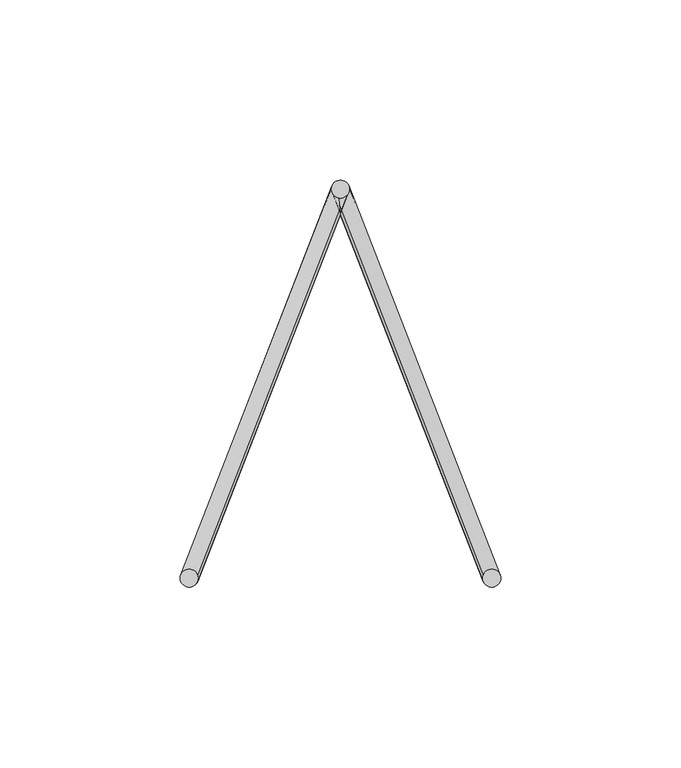
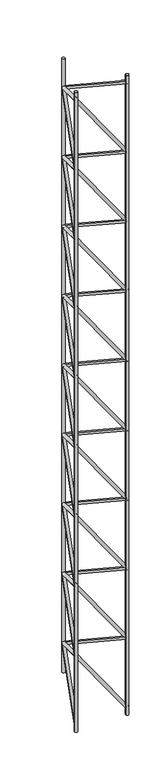
"""IFC4 building model written with IfcOpenShell, lengths in millimetres: proxy geometry, Pre-fab. (Vigota 3 - Pano 8)."""

from ifc_helpers import new_model, si_unit, point, frame, frame_2d, origin, origin_with_axes, origin_2d, place, context, project, spatial, circle_curve, trimmed, segment, composite_curve, outline, extrude, source, transform, mapped, element, save


def structural_framing_089a5535(model_context):
    return source(origin(), model_context, "Body", "SweptSolid", [
        extrude(outline(composite_curve([segment(trimmed(circle_curve(origin_2d(), 2.5), [point((2.5, 0.0))], [point((-2.5, 0.0))], False, "CARTESIAN"), True, "CONTINUOUS"), segment(trimmed(circle_curve(origin_2d(), 2.5), [point((-2.5, 0.0))], [point((2.5, 0.0))], False, "CARTESIAN"), True, "CONTINUOUS")], self_intersect=False)), origin_with_axes(), (0.0, 0.0, 1.0), 1105.691264),
        extrude(outline(composite_curve([segment(trimmed(circle_curve(frame_2d((-42.0, 108.0)), 2.5), [point((-39.5, 108.0))], [point((-44.5, 108.0))], False, "CARTESIAN"), True, "CONTINUOUS"), segment(trimmed(circle_curve(frame_2d((-42.0, 108.0)), 2.5), [point((-44.5, 108.0))], [point((-39.5, 108.0))], False, "CARTESIAN"), True, "CONTINUOUS")], self_intersect=False)), frame((0.0, 0.0, 22.8456318), z_axis=(0.0, 0.0, 1.0), x_axis=(1.0, 0.0, 0.0)), (0.0, 0.0, 1.0), 1060.0),
        extrude(outline(composite_curve([segment(trimmed(circle_curve(origin_2d(), 2.5), [point((2.5, 0.0))], [point((-2.5, 0.0))], False, "CARTESIAN"), True, "CONTINUOUS"), segment(trimmed(circle_curve(origin_2d(), 2.5), [point((-2.5, 0.0))], [point((2.5, 0.0))], False, "CARTESIAN"), True, "CONTINUOUS")], self_intersect=False)), frame((0.0, 0.0, 12.8456318), z_axis=(-0.3218603428886276, 0.8276408817707567, 0.4598004898837537), x_axis=(0.8192319205108605, -3.936835275445103e-11, 0.5734623443750141)), (0.0, 0.0, 1.0), 130.491379),
        extrude(outline(composite_curve([segment(trimmed(circle_curve(origin_2d(), 2.5), [point((2.5, 0.0))], [point((-2.5, 0.0))], False, "CARTESIAN"), True, "CONTINUOUS"), segment(trimmed(circle_curve(origin_2d(), 2.5), [point((-2.5, 0.0))], [point((2.5, 0.0))], False, "CARTESIAN"), True, "CONTINUOUS")], self_intersect=False)), frame((-42.0, 108.0, 72.8456318), z_axis=(0.3218603428886276, -0.8276408817707567, 0.4598004898837537), x_axis=(0.8192319205108605, -3.936835275445103e-11, -0.5734623443750141)), (0.0, 0.0, 1.0), 130.491379),
        extrude(outline(composite_curve([segment(trimmed(circle_curve(origin_2d(), 2.5), [point((2.5, 0.0))], [point((-2.5, 0.0))], False, "CARTESIAN"), True, "CONTINUOUS"), segment(trimmed(circle_curve(origin_2d(), 2.5), [point((-2.5, 0.0))], [point((2.5, 0.0))], False, "CARTESIAN"), True, "CONTINUOUS")], self_intersect=False)), frame((0.0, 0.0, 132.8456318), z_axis=(-0.3218603428886276, 0.8276408817707567, 0.4598004898837537), x_axis=(0.8192319205108605, -3.936835275445103e-11, 0.5734623443750141)), (0.0, 0.0, 1.0), 130.491379),
        extrude(outline(composite_curve([segment(trimmed(circle_curve(origin_2d(), 2.5), [point((2.5, 0.0))], [point((-2.5, 0.0))], False, "CARTESIAN"), True, "CONTINUOUS"), segment(trimmed(circle_curve(origin_2d(), 2.5), [point((-2.5, 0.0))], [point((2.5, 0.0))], False, "CARTESIAN"), True, "CONTINUOUS")], self_intersect=False)), frame((-42.0, 108.0, 192.8456318), z_axis=(0.3218603428886276, -0.8276408817707567, 0.4598004898837537), x_axis=(0.8192319205108605, -3.936835275445103e-11, -0.5734623443750141)), (0.0, 0.0, 1.0), 130.491379),
        extrude(outline(composite_curve([segment(trimmed(circle_curve(origin_2d(), 2.5), [point((2.5, 0.0))], [point((-2.5, 0.0))], False, "CARTESIAN"), True, "CONTINUOUS"), segment(trimmed(circle_curve(origin_2d(), 2.5), [point((-2.5, 0.0))], [point((2.5, 0.0))], False, "CARTESIAN"), True, "CONTINUOUS")], self_intersect=False)), frame((0.0, 0.0, 252.8456318), z_axis=(-0.3218603428886276, 0.8276408817707567, 0.4598004898837537), x_axis=(0.8192319205108605, -3.936835275445103e-11, 0.5734623443750141)), (0.0, 0.0, 1.0), 130.491379),
        extrude(outline(composite_curve([segment(trimmed(circle_curve(origin_2d(), 2.5), [point((2.5, 0.0))], [point((-2.5, 0.0))], False, "CARTESIAN"), True, "CONTINUOUS"), segment(trimmed(circle_curve(origin_2d(), 2.5), [point((-2.5, 0.0))], [point((2.5, 0.0))], False, "CARTESIAN"), True, "CONTINUOUS")], self_intersect=False)), frame((-42.0, 108.0, 312.8456318), z_axis=(0.3218603428886276, -0.8276408817707567, 0.4598004898837537), x_axis=(0.8192319205108605, -3.936835275445103e-11, -0.5734623443750141)), (0.0, 0.0, 1.0), 130.491379),
        extrude(outline(composite_curve([segment(trimmed(circle_curve(origin_2d(), 2.5), [point((2.5, 0.0))], [point((-2.5, 0.0))], False, "CARTESIAN"), True, "CONTINUOUS"), segment(trimmed(circle_curve(origin_2d(), 2.5), [point((-2.5, 0.0))], [point((2.5, 0.0))], False, "CARTESIAN"), True, "CONTINUOUS")], self_intersect=False)), frame((0.0, 0.0, 372.8456318), z_axis=(-0.3218603428886276, 0.8276408817707567, 0.4598004898837537), x_axis=(0.8192319205108605, -3.936835275445103e-11, 0.5734623443750141)), (0.0, 0.0, 1.0), 130.491379),
        extrude(outline(composite_curve([segment(trimmed(circle_curve(origin_2d(), 2.5), [point((2.5, 0.0))], [point((-2.5, 0.0))], False, "CARTESIAN"), True, "CONTINUOUS"), segment(trimmed(circle_curve(origin_2d(), 2.5), [point((-2.5, 0.0))], [point((2.5, 0.0))], False, "CARTESIAN"), True, "CONTINUOUS")], self_intersect=False)), frame((-42.0, 108.0, 432.8456318), z_axis=(0.3218603428886276, -0.8276408817707567, 0.4598004898837537), x_axis=(0.8192319205108605, -3.936835275445103e-11, -0.5734623443750141)), (0.0, 0.0, 1.0), 130.491379),
        extrude(outline(composite_curve([segment(trimmed(circle_curve(origin_2d(), 2.5), [point((2.5, 0.0))], [point((-2.5, 0.0))], False, "CARTESIAN"), True, "CONTINUOUS"), segment(trimmed(circle_curve(origin_2d(), 2.5), [point((-2.5, 0.0))], [point((2.5, 0.0))], False, "CARTESIAN"), True, "CONTINUOUS")], self_intersect=False)), frame((0.0, 0.0, 492.8456318), z_axis=(-0.3218603428886276, 0.8276408817707567, 0.4598004898837537), x_axis=(0.8192319205108605, -3.936835275445103e-11, 0.5734623443750141)), (0.0, 0.0, 1.0), 130.491379),
        extrude(outline(composite_curve([segment(trimmed(circle_curve(origin_2d(), 2.5), [point((2.5, 0.0))], [point((-2.5, 0.0))], False, "CARTESIAN"), True, "CONTINUOUS"), segment(trimmed(circle_curve(origin_2d(), 2.5), [point((-2.5, 0.0))], [point((2.5, 0.0))], False, "CARTESIAN"), True, "CONTINUOUS")], self_intersect=False)), frame((-42.0, 108.0, 552.8456318), z_axis=(0.3218603428886276, -0.8276408817707567, 0.4598004898837537), x_axis=(0.8192319205108605, -3.936835275445103e-11, -0.5734623443750141)), (0.0, 0.0, 1.0), 130.491379),
        extrude(outline(composite_curve([segment(trimmed(circle_curve(origin_2d(), 2.5), [point((2.5, 0.0))], [point((-2.5, 0.0))], False, "CARTESIAN"), True, "CONTINUOUS"), segment(trimmed(circle_curve(origin_2d(), 2.5), [point((-2.5, 0.0))], [point((2.5, 0.0))], False, "CARTESIAN"), True, "CONTINUOUS")], self_intersect=False)), frame((0.0, 0.0, 612.8456318), z_axis=(-0.3218603428886276, 0.8276408817707567, 0.4598004898837537), x_axis=(0.8192319205108605, -3.936835275445103e-11, 0.5734623443750141)), (0.0, 0.0, 1.0), 130.491379),
        extrude(outline(composite_curve([segment(trimmed(circle_curve(origin_2d(), 2.5), [point((2.5, 0.0))], [point((-2.5, 0.0))], False, "CARTESIAN"), True, "CONTINUOUS"), segment(trimmed(circle_curve(origin_2d(), 2.5), [point((-2.5, 0.0))], [point((2.5, 0.0))], False, "CARTESIAN"), True, "CONTINUOUS")], self_intersect=False)), frame((-42.0, 108.0, 672.8456318), z_axis=(0.3218603428886276, -0.8276408817707567, 0.4598004898837537), x_axis=(0.8192319205108605, -3.936835275445103e-11, -0.5734623443750141)), (0.0, 0.0, 1.0), 130.491379),
        extrude(outline(composite_curve([segment(trimmed(circle_curve(origin_2d(), 2.5), [point((2.5, 0.0))], [point((-2.5, 0.0))], False, "CARTESIAN"), True, "CONTINUOUS"), segment(trimmed(circle_curve(origin_2d(), 2.5), [point((-2.5, 0.0))], [point((2.5, 0.0))], False, "CARTESIAN"), True, "CONTINUOUS")], self_intersect=False)), frame((0.0, 0.0, 732.8456318), z_axis=(-0.3218603428886276, 0.8276408817707567, 0.4598004898837537), x_axis=(0.8192319205108605, -3.936835275445103e-11, 0.5734623443750141)), (0.0, 0.0, 1.0), 130.491379),
        extrude(outline(composite_curve([segment(trimmed(circle_curve(origin_2d(), 2.5), [point((2.5, 0.0))], [point((-2.5, 0.0))], False, "CARTESIAN"), True, "CONTINUOUS"), segment(trimmed(circle_curve(origin_2d(), 2.5), [point((-2.5, 0.0))], [point((2.5, 0.0))], False, "CARTESIAN"), True, "CONTINUOUS")], self_intersect=False)), frame((-42.0, 108.0, 792.8456318), z_axis=(0.3218603428886276, -0.8276408817707567, 0.4598004898837537), x_axis=(0.8192319205108605, -3.936835275445103e-11, -0.5734623443750141)), (0.0, 0.0, 1.0), 130.491379),
        extrude(outline(composite_curve([segment(trimmed(circle_curve(origin_2d(), 2.5), [point((2.5, 0.0))], [point((-2.5, 0.0))], False, "CARTESIAN"), True, "CONTINUOUS"), segment(trimmed(circle_curve(origin_2d(), 2.5), [point((-2.5, 0.0))], [point((2.5, 0.0))], False, "CARTESIAN"), True, "CONTINUOUS")], self_intersect=False)), frame((0.0, 0.0, 852.8456318), z_axis=(-0.3218603428886276, 0.8276408817707567, 0.4598004898837537), x_axis=(0.8192319205108605, -3.936835275445103e-11, 0.5734623443750141)), (0.0, 0.0, 1.0), 130.491379),
        extrude(outline(composite_curve([segment(trimmed(circle_curve(origin_2d(), 2.5), [point((2.5, 0.0))], [point((-2.5, 0.0))], False, "CARTESIAN"), True, "CONTINUOUS"), segment(trimmed(circle_curve(origin_2d(), 2.5), [point((-2.5, 0.0))], [point((2.5, 0.0))], False, "CARTESIAN"), True, "CONTINUOUS")], self_intersect=False)), frame((-42.0, 108.0, 912.8456318), z_axis=(0.3218603428886276, -0.8276408817707567, 0.4598004898837537), x_axis=(0.8192319205108605, -3.936835275445103e-11, -0.5734623443750141)), (0.0, 0.0, 1.0), 130.491379),
        extrude(outline(composite_curve([segment(trimmed(circle_curve(origin_2d(), 2.5), [point((2.5, 0.0))], [point((-2.5, 0.0))], False, "CARTESIAN"), True, "CONTINUOUS"), segment(trimmed(circle_curve(origin_2d(), 2.5), [point((-2.5, 0.0))], [point((2.5, 0.0))], False, "CARTESIAN"), True, "CONTINUOUS")], self_intersect=False)), frame((0.0, 0.0, 972.8456318), z_axis=(-0.3218603428886276, 0.8276408817707567, 0.4598004898837537), x_axis=(0.8192319205108605, -3.936835275445103e-11, 0.5734623443750141)), (0.0, 0.0, 1.0), 130.491379),
        extrude(outline(composite_curve([segment(trimmed(circle_curve(origin_2d(), 2.5), [point((2.5, 0.0))], [point((-2.5, 0.0))], False, "CARTESIAN"), True, "CONTINUOUS"), segment(trimmed(circle_curve(origin_2d(), 2.5), [point((-2.5, 0.0))], [point((2.5, 0.0))], False, "CARTESIAN"), True, "CONTINUOUS")], self_intersect=False)), frame((-42.0, 108.0, 1032.845632), z_axis=(0.3218603428886276, -0.8276408817707567, 0.4598004898837537), x_axis=(0.8192319205108605, -3.936835275445103e-11, -0.5734623443750141)), (0.0, 0.0, 1.0), 130.491379),
        extrude(outline(composite_curve([segment(trimmed(circle_curve(frame_2d((-84.0, 0.0)), 2.5), [point((-81.5, 0.0))], [point((-86.5, 0.0))], False, "CARTESIAN"), True, "CONTINUOUS"), segment(trimmed(circle_curve(frame_2d((-84.0, 0.0)), 2.5), [point((-86.5, 0.0))], [point((-81.5, 0.0))], False, "CARTESIAN"), True, "CONTINUOUS")], self_intersect=False)), origin_with_axes(), (0.0, 0.0, 1.0), 1105.691264),
        extrude(outline(composite_curve([segment(trimmed(circle_curve(origin_2d(), 2.5), [point((2.5, 0.0))], [point((-2.5, 0.0))], False, "CARTESIAN"), True, "CONTINUOUS"), segment(trimmed(circle_curve(origin_2d(), 2.5), [point((-2.5, 0.0))], [point((2.5, 0.0))], False, "CARTESIAN"), True, "CONTINUOUS")], self_intersect=False)), frame((-84.0, 0.0, 12.8456318), z_axis=(0.3218603428886276, 0.8276408817707567, 0.4598004898837537), x_axis=(0.8192319205108605, 3.936835275445103e-11, -0.5734623443750141)), (0.0, 0.0, 1.0), 130.491379),
        extrude(outline(composite_curve([segment(trimmed(circle_curve(origin_2d(), 2.5), [point((2.5, 0.0))], [point((-2.5, 0.0))], False, "CARTESIAN"), True, "CONTINUOUS"), segment(trimmed(circle_curve(origin_2d(), 2.5), [point((-2.5, 0.0))], [point((2.5, 0.0))], False, "CARTESIAN"), True, "CONTINUOUS")], self_intersect=False)), frame((-42.0, 108.0, 72.8456318), z_axis=(-0.3218603428886276, -0.8276408817707567, 0.4598004898837537), x_axis=(0.8192319205108605, 3.936835275445103e-11, 0.5734623443750141)), (0.0, 0.0, 1.0), 130.491379),
        extrude(outline(composite_curve([segment(trimmed(circle_curve(origin_2d(), 2.5), [point((2.5, 0.0))], [point((-2.5, 0.0))], False, "CARTESIAN"), True, "CONTINUOUS"), segment(trimmed(circle_curve(origin_2d(), 2.5), [point((-2.5, 0.0))], [point((2.5, 0.0))], False, "CARTESIAN"), True, "CONTINUOUS")], self_intersect=False)), frame((-84.0, 0.0, 132.8456318), z_axis=(0.3218603428886276, 0.8276408817707567, 0.4598004898837537), x_axis=(0.8192319205108605, 3.936835275445103e-11, -0.5734623443750141)), (0.0, 0.0, 1.0), 130.491379),
        extrude(outline(composite_curve([segment(trimmed(circle_curve(origin_2d(), 2.5), [point((2.5, 0.0))], [point((-2.5, 0.0))], False, "CARTESIAN"), True, "CONTINUOUS"), segment(trimmed(circle_curve(origin_2d(), 2.5), [point((-2.5, 0.0))], [point((2.5, 0.0))], False, "CARTESIAN"), True, "CONTINUOUS")], self_intersect=False)), frame((-42.0, 108.0, 192.8456318), z_axis=(-0.3218603428886276, -0.8276408817707567, 0.4598004898837537), x_axis=(0.8192319205108605, 3.936835275445103e-11, 0.5734623443750141)), (0.0, 0.0, 1.0), 130.491379),
        extrude(outline(composite_curve([segment(trimmed(circle_curve(origin_2d(), 2.5), [point((2.5, 0.0))], [point((-2.5, 0.0))], False, "CARTESIAN"), True, "CONTINUOUS"), segment(trimmed(circle_curve(origin_2d(), 2.5), [point((-2.5, 0.0))], [point((2.5, 0.0))], False, "CARTESIAN"), True, "CONTINUOUS")], self_intersect=False)), frame((-84.0, 0.0, 252.8456318), z_axis=(0.3218603428886276, 0.8276408817707567, 0.4598004898837537), x_axis=(0.8192319205108605, 3.936835275445103e-11, -0.5734623443750141)), (0.0, 0.0, 1.0), 130.491379),
        extrude(outline(composite_curve([segment(trimmed(circle_curve(origin_2d(), 2.5), [point((2.5, 0.0))], [point((-2.5, 0.0))], False, "CARTESIAN"), True, "CONTINUOUS"), segment(trimmed(circle_curve(origin_2d(), 2.5), [point((-2.5, 0.0))], [point((2.5, 0.0))], False, "CARTESIAN"), True, "CONTINUOUS")], self_intersect=False)), frame((-42.0, 108.0, 312.8456318), z_axis=(-0.3218603428886276, -0.8276408817707567, 0.4598004898837537), x_axis=(0.8192319205108605, 3.936835275445103e-11, 0.5734623443750141)), (0.0, 0.0, 1.0), 130.491379),
        extrude(outline(composite_curve([segment(trimmed(circle_curve(origin_2d(), 2.5), [point((2.5, 0.0))], [point((-2.5, 0.0))], False, "CARTESIAN"), True, "CONTINUOUS"), segment(trimmed(circle_curve(origin_2d(), 2.5), [point((-2.5, 0.0))], [point((2.5, 0.0))], False, "CARTESIAN"), True, "CONTINUOUS")], self_intersect=False)), frame((-84.0, 0.0, 372.8456318), z_axis=(0.3218603428886276, 0.8276408817707567, 0.4598004898837537), x_axis=(0.8192319205108605, 3.936835275445103e-11, -0.5734623443750141)), (0.0, 0.0, 1.0), 130.491379),
        extrude(outline(composite_curve([segment(trimmed(circle_curve(origin_2d(), 2.5), [point((2.5, 0.0))], [point((-2.5, 0.0))], False, "CARTESIAN"), True, "CONTINUOUS"), segment(trimmed(circle_curve(origin_2d(), 2.5), [point((-2.5, 0.0))], [point((2.5, 0.0))], False, "CARTESIAN"), True, "CONTINUOUS")], self_intersect=False)), frame((-42.0, 108.0, 432.8456318), z_axis=(-0.3218603428886276, -0.8276408817707567, 0.4598004898837537), x_axis=(0.8192319205108605, 3.936835275445103e-11, 0.5734623443750141)), (0.0, 0.0, 1.0), 130.491379),
        extrude(outline(composite_curve([segment(trimmed(circle_curve(origin_2d(), 2.5), [point((2.5, 0.0))], [point((-2.5, 0.0))], False, "CARTESIAN"), True, "CONTINUOUS"), segment(trimmed(circle_curve(origin_2d(), 2.5), [point((-2.5, 0.0))], [point((2.5, 0.0))], False, "CARTESIAN"), True, "CONTINUOUS")], self_intersect=False)), frame((-84.0, 0.0, 492.8456318), z_axis=(0.3218603428886276, 0.8276408817707567, 0.4598004898837537), x_axis=(0.8192319205108605, 3.936835275445103e-11, -0.5734623443750141)), (0.0, 0.0, 1.0), 130.491379),
        extrude(outline(composite_curve([segment(trimmed(circle_curve(origin_2d(), 2.5), [point((2.5, 0.0))], [point((-2.5, 0.0))], False, "CARTESIAN"), True, "CONTINUOUS"), segment(trimmed(circle_curve(origin_2d(), 2.5), [point((-2.5, 0.0))], [point((2.5, 0.0))], False, "CARTESIAN"), True, "CONTINUOUS")], self_intersect=False)), frame((-42.0, 108.0, 552.8456318), z_axis=(-0.3218603428886276, -0.8276408817707567, 0.4598004898837537), x_axis=(0.8192319205108605, 3.936835275445103e-11, 0.5734623443750141)), (0.0, 0.0, 1.0), 130.491379),
        extrude(outline(composite_curve([segment(trimmed(circle_curve(origin_2d(), 2.5), [point((2.5, 0.0))], [point((-2.5, 0.0))], False, "CARTESIAN"), True, "CONTINUOUS"), segment(trimmed(circle_curve(origin_2d(), 2.5), [point((-2.5, 0.0))], [point((2.5, 0.0))], False, "CARTESIAN"), True, "CONTINUOUS")], self_intersect=False)), frame((-84.0, 0.0, 612.8456318), z_axis=(0.3218603428886276, 0.8276408817707567, 0.4598004898837537), x_axis=(0.8192319205108605, 3.936835275445103e-11, -0.5734623443750141)), (0.0, 0.0, 1.0), 130.491379),
        extrude(outline(composite_curve([segment(trimmed(circle_curve(origin_2d(), 2.5), [point((2.5, 0.0))], [point((-2.5, 0.0))], False, "CARTESIAN"), True, "CONTINUOUS"), segment(trimmed(circle_curve(origin_2d(), 2.5), [point((-2.5, 0.0))], [point((2.5, 0.0))], False, "CARTESIAN"), True, "CONTINUOUS")], self_intersect=False)), frame((-42.0, 108.0, 672.8456318), z_axis=(-0.3218603428886276, -0.8276408817707567, 0.4598004898837537), x_axis=(0.8192319205108605, 3.936835275445103e-11, 0.5734623443750141)), (0.0, 0.0, 1.0), 130.491379),
        extrude(outline(composite_curve([segment(trimmed(circle_curve(origin_2d(), 2.5), [point((2.5, 0.0))], [point((-2.5, 0.0))], False, "CARTESIAN"), True, "CONTINUOUS"), segment(trimmed(circle_curve(origin_2d(), 2.5), [point((-2.5, 0.0))], [point((2.5, 0.0))], False, "CARTESIAN"), True, "CONTINUOUS")], self_intersect=False)), frame((-84.0, 0.0, 732.8456318), z_axis=(0.3218603428886276, 0.8276408817707567, 0.4598004898837537), x_axis=(0.8192319205108605, 3.936835275445103e-11, -0.5734623443750141)), (0.0, 0.0, 1.0), 130.491379),
        extrude(outline(composite_curve([segment(trimmed(circle_curve(origin_2d(), 2.5), [point((2.5, 0.0))], [point((-2.5, 0.0))], False, "CARTESIAN"), True, "CONTINUOUS"), segment(trimmed(circle_curve(origin_2d(), 2.5), [point((-2.5, 0.0))], [point((2.5, 0.0))], False, "CARTESIAN"), True, "CONTINUOUS")], self_intersect=False)), frame((-42.0, 108.0, 792.8456318), z_axis=(-0.3218603428886276, -0.8276408817707567, 0.4598004898837537), x_axis=(0.8192319205108605, 3.936835275445103e-11, 0.5734623443750141)), (0.0, 0.0, 1.0), 130.491379),
        extrude(outline(composite_curve([segment(trimmed(circle_curve(origin_2d(), 2.5), [point((2.5, 0.0))], [point((-2.5, 0.0))], False, "CARTESIAN"), True, "CONTINUOUS"), segment(trimmed(circle_curve(origin_2d(), 2.5), [point((-2.5, 0.0))], [point((2.5, 0.0))], False, "CARTESIAN"), True, "CONTINUOUS")], self_intersect=False)), frame((-84.0, 0.0, 852.8456318), z_axis=(0.3218603428886276, 0.8276408817707567, 0.4598004898837537), x_axis=(0.8192319205108605, 3.936835275445103e-11, -0.5734623443750141)), (0.0, 0.0, 1.0), 130.491379),
        extrude(outline(composite_curve([segment(trimmed(circle_curve(origin_2d(), 2.5), [point((2.5, 0.0))], [point((-2.5, 0.0))], False, "CARTESIAN"), True, "CONTINUOUS"), segment(trimmed(circle_curve(origin_2d(), 2.5), [point((-2.5, 0.0))], [point((2.5, 0.0))], False, "CARTESIAN"), True, "CONTINUOUS")], self_intersect=False)), frame((-42.0, 108.0, 912.8456318), z_axis=(-0.3218603428886276, -0.8276408817707567, 0.4598004898837537), x_axis=(0.8192319205108605, 3.936835275445103e-11, 0.5734623443750141)), (0.0, 0.0, 1.0), 130.491379),
        extrude(outline(composite_curve([segment(trimmed(circle_curve(origin_2d(), 2.5), [point((2.5, 0.0))], [point((-2.5, 0.0))], False, "CARTESIAN"), True, "CONTINUOUS"), segment(trimmed(circle_curve(origin_2d(), 2.5), [point((-2.5, 0.0))], [point((2.5, 0.0))], False, "CARTESIAN"), True, "CONTINUOUS")], self_intersect=False)), frame((-84.0, 0.0, 972.8456318), z_axis=(0.3218603428886276, 0.8276408817707567, 0.4598004898837537), x_axis=(0.8192319205108605, 3.936835275445103e-11, -0.5734623443750141)), (0.0, 0.0, 1.0), 130.491379),
        extrude(outline(composite_curve([segment(trimmed(circle_curve(origin_2d(), 2.5), [point((2.5, 0.0))], [point((-2.5, 0.0))], False, "CARTESIAN"), True, "CONTINUOUS"), segment(trimmed(circle_curve(origin_2d(), 2.5), [point((-2.5, 0.0))], [point((2.5, 0.0))], False, "CARTESIAN"), True, "CONTINUOUS")], self_intersect=False)), frame((-42.0, 108.0, 1032.845632), z_axis=(-0.3218603428886276, -0.8276408817707567, 0.4598004898837537), x_axis=(0.8192319205108605, 3.936835275445103e-11, 0.5734623443750141)), (0.0, 0.0, 1.0), 130.491379),
    ])


if __name__ == "__main__":
    model = new_model("IFC4")
    model_context = context("Model", 3, world=origin())
    ifc_project = project(units=[si_unit("LENGTHUNIT", "METRE", prefix="MILLI")], contexts=[model_context])
    site = spatial("IfcSite", under=ifc_project)
    building = spatial("IfcBuilding", under=site)
    placement = place(None, origin())
    structural_framing_shape = structural_framing_089a5535(model_context)
    element("IfcBuildingElementProxy", 1, Name="Pre-fab. (Vigota 3 - Pano 8)", ObjectType="Pre-fab. (Vigota 3 - Pano 8)", at=placement, inside=building, context=model_context, shape_type="MappedRepresentation", body=[
        mapped(structural_framing_shape, transform((0.0, 0.0, 0.0), x_axis=(1.0, 0.0, 0.0), y_axis=(0.0, 1.0, 0.0), z_axis=(0.0, 0.0, 1.0))),
    ])
    save(model, "model.ifc")

# Revit data of these elements
# Element 1 (IfcBuildingElementProxy, "Pre-fab. (Vigota 3 - Pano 8)")
#   Materials on its faces: "Aço"
# Materials
#   "Aço": class "Metal", colour RGB 120 120 120, transparency 0, Description = "Aço estrutural A36 grau, ASTM B, acabamento laminado", Cost = 0
